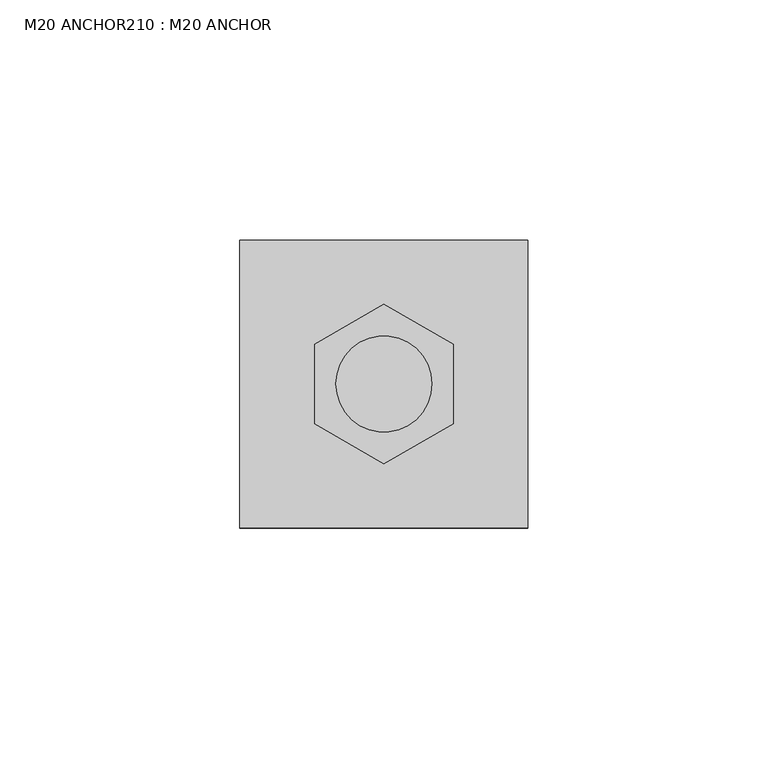
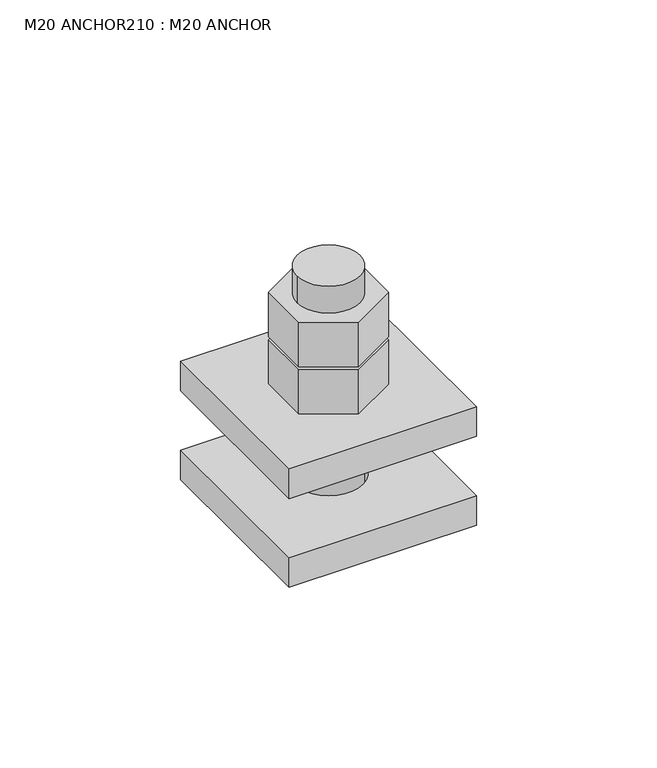
"""IFC4 building model written with IfcOpenShell, lengths in millimetres: fastener geometry, M20 ANCHOR210 : M20 ANCHOR."""

import ifcopenshell
import ifcopenshell.guid

model = None  # the IFC model being written
_history = None  # IfcOwnerHistory: only IFC2X3 demands one
_inside = {}  # id of a spatial element -> (the spatial element, [elements in it])
_under = {}  # id of a project, library or spatial element -> (it, [spatial elements below it])
_declared = {}  # id of a project -> (the project, [libraries it declares])
_typed = {}  # id of a type object -> (the type object, [elements of that type])
_made_of = {}  # id of a material, layer set ... -> (it, [elements and type objects made of it])


def new_model(schema):
    """Start an empty IFC model of exactly this schema.

    Asked for "IFC4X3", IfcOpenShell would pick the latest addendum, in which some entities
    have other attributes; the version numbers below select the first issue.
    IFC2X3 requires an IfcOwnerHistory on every rooted entity: one is made here for all.
    """
    global model, _history
    if schema == "IFC4X3":
        model = ifcopenshell.file(schema_version=(4, 3, 0, 0))
    else:
        model = ifcopenshell.file(schema=schema)
    _inside.clear()
    _under.clear()
    _declared.clear()
    _typed.clear()
    _made_of.clear()
    _history = None
    if model.schema == "IFC2X3":
        org = make("IfcOrganization", Name="unknown")
        user = make(
            "IfcPersonAndOrganization",
            ThePerson=make("IfcPerson", FamilyName="unknown"),
            TheOrganization=org,
        )
        app = make(
            "IfcApplication",
            ApplicationDeveloper=org,
            Version="unknown",
            ApplicationFullName="unknown",
            ApplicationIdentifier="unknown",
        )
        _history = make(
            "IfcOwnerHistory",
            OwningUser=user,
            OwningApplication=app,
            ChangeAction="ADDED",
            CreationDate=0,
        )
    return model


def make(cls, **values):
    """One entity of the class cls with the attributes given. An attribute that is None is left unset."""
    return model.create_entity(
        cls, **{name: value for name, value in values.items() if value is not None}
    )


def rooted(cls, **values):
    """An entity with a GlobalId (a new one), such as an element, a storey or a relation."""
    return make(cls, GlobalId=ifcopenshell.guid.new(), OwnerHistory=_history, **values)


def si_unit(unit_type, name, prefix=None):
    """IfcSIUnit, for example si_unit("LENGTHUNIT", "METRE", prefix="MILLI")."""
    return make("IfcSIUnit", UnitType=unit_type, Prefix=prefix, Name=name)


def assignment(units):
    """IfcUnitAssignment: the units of a project."""
    return None if units is None else make("IfcUnitAssignment", Units=units)


def point(xyz):
    """IfcCartesianPoint."""
    return None if xyz is None else make("IfcCartesianPoint", Coordinates=xyz)


def direction(xyz):
    """IfcDirection."""
    return None if xyz is None else make("IfcDirection", DirectionRatios=xyz)


def frame(location, z_axis=None, x_axis=None):
    """IfcAxis2Placement3D, a coordinate frame: its origin and axes. An axis left out is left unset."""
    return make(
        "IfcAxis2Placement3D",
        Location=point(location),
        Axis=direction(z_axis),
        RefDirection=direction(x_axis),
    )


def frame_2d(location, x_axis=None):
    """IfcAxis2Placement2D, a coordinate frame in the plane: its origin and x axis."""
    return make(
        "IfcAxis2Placement2D", Location=point(location), RefDirection=direction(x_axis)
    )


def origin():
    """The frame at (0, 0, 0) with its axes left unset."""
    return frame((0.0, 0.0, 0.0))


def place(relative_to, where):
    """IfcLocalPlacement: puts the frame where relative to a parent placement (None: the world)."""
    return make(
        "IfcLocalPlacement", PlacementRelTo=relative_to, RelativePlacement=where
    )


def context(
    kind, dimensions, precision=None, world=None, true_north=None, identifier=None
):
    """IfcGeometricRepresentationContext, for example the 3D "Model" context."""
    return make(
        "IfcGeometricRepresentationContext",
        ContextIdentifier=identifier,
        ContextType=kind,
        CoordinateSpaceDimension=dimensions,
        Precision=precision,
        WorldCoordinateSystem=world,
        TrueNorth=true_north,
    )


def project(units=None, contexts=None):
    """IfcProject with its units and contexts."""
    return rooted(
        "IfcProject",
        Name="project",
        RepresentationContexts=contexts,
        UnitsInContext=assignment(units),
    )


def spatial(cls, under=None, at=None, **own):
    """A site, building, storey or space (cls), placed at a placement, below another one or the project."""
    s = rooted(cls, ObjectPlacement=at, **own)
    if under is not None:
        _under.setdefault(under.id(), (under, []))[1].append(s)
    return s


def polyline(points):
    """IfcPolyline through the points."""
    return make("IfcPolyline", Points=[point(p) for p in points])


def circle_curve(where, radius):
    """IfcCircle in the frame where."""
    return make("IfcCircle", Position=where, Radius=radius)


def trimmed(basis, trim1, trim2, sense, master):
    """IfcTrimmedCurve: the piece of a basis curve between two trims."""
    return make(
        "IfcTrimmedCurve",
        BasisCurve=basis,
        Trim1=trim1,
        Trim2=trim2,
        SenseAgreement=sense,
        MasterRepresentation=master,
    )


def segment(curve, same_sense, transition):
    """IfcCompositeCurveSegment."""
    return make(
        "IfcCompositeCurveSegment",
        Transition=transition,
        SameSense=same_sense,
        ParentCurve=curve,
    )


def composite_curve(segments, self_intersect=None):
    """IfcCompositeCurve: segments joined end to end."""
    return make("IfcCompositeCurve", Segments=segments, SelfIntersect=self_intersect)


def outline(outer, holes=None, kind="AREA"):
    """IfcArbitraryClosedProfileDef: a profile drawn as a closed curve; with holes, ...WithVoids."""
    if holes is None:
        return make("IfcArbitraryClosedProfileDef", ProfileType=kind, OuterCurve=outer)
    return make(
        "IfcArbitraryProfileDefWithVoids",
        ProfileType=kind,
        OuterCurve=outer,
        InnerCurves=holes,
    )


def extrude(swept, where, along, depth):
    """IfcExtrudedAreaSolid: the profile swept, set in the frame where, extruded along a direction by depth."""
    return make(
        "IfcExtrudedAreaSolid",
        SweptArea=swept,
        Position=where,
        ExtrudedDirection=direction(along),
        Depth=depth,
    )


def shape(context_of_items, identifier, shape_type, items):
    """IfcShapeRepresentation: the items that make up one representation, for example the "Body"."""
    return make(
        "IfcShapeRepresentation",
        ContextOfItems=context_of_items,
        RepresentationIdentifier=identifier,
        RepresentationType=shape_type,
        Items=items,
    )


def source(mapping_origin, context_of_items, identifier, shape_type, items):
    """IfcRepresentationMap: a shape defined once, which mapped items show again and again."""
    return make(
        "IfcRepresentationMap",
        MappingOrigin=mapping_origin,
        MappedRepresentation=shape(context_of_items, identifier, shape_type, items),
    )


def transform(
    local_origin,
    x_axis=None,
    y_axis=None,
    z_axis=None,
    scale=None,
    scale2=None,
    scale3=None,
    uniform=True,
):
    """IfcCartesianTransformationOperator3D, or its non-uniform kind. x_axis, y_axis, z_axis: its Axis1, 2, 3."""
    if uniform:
        return make(
            "IfcCartesianTransformationOperator3D",
            Axis1=direction(x_axis),
            Axis2=direction(y_axis),
            LocalOrigin=point(local_origin),
            Scale=scale,
            Axis3=direction(z_axis),
        )
    return make(
        "IfcCartesianTransformationOperator3DnonUniform",
        Axis1=direction(x_axis),
        Axis2=direction(y_axis),
        LocalOrigin=point(local_origin),
        Scale=scale,
        Axis3=direction(z_axis),
        Scale2=scale2,
        Scale3=scale3,
    )


def mapped(mapping_source, mapping_target):
    """IfcMappedItem: shows the shape of a source again, moved by a transform."""
    return make(
        "IfcMappedItem", MappingSource=mapping_source, MappingTarget=mapping_target
    )


def made_of(thing, what):
    """Note that an element or type object is made of a material, layer set ...; save() writes the relation."""
    if what is not None:
        _made_of.setdefault(what.id(), (what, []))[1].append(thing)
    return thing


def element(
    cls,
    number,
    at=None,
    inside=None,
    cuts=None,
    type_object=None,
    material=None,
    context=None,
    identifier="Body",
    shape_type=None,
    held_by="IfcProductDefinitionShape",
    body=None,
    shapes=None,
    **own,
):
    """One element of the class cls, such as IfcWall. Its Tag is "e" and its number.

    at: its placement. inside: the storey or other place that contains it. cuts: it is an
    opening in that element (IfcRelVoidsElement). A single representation is given by context,
    identifier, shape_type and body (its items); several are given by shapes. held_by: the class
    of the entity that holds the representations. save() writes the other relations.
    """
    e = rooted(cls, Tag="e%d" % number, ObjectPlacement=at, **own)
    if body is not None:
        shapes = [shape(context, identifier, shape_type, body)]
    if shapes is not None:
        e.Representation = make(held_by, Representations=shapes)
    if inside is not None:
        _inside.setdefault(inside.id(), (inside, []))[1].append(e)
    if cuts is not None:
        rooted(
            "IfcRelVoidsElement", RelatingBuildingElement=cuts, RelatedOpeningElement=e
        )
    if type_object is not None:
        _typed.setdefault(type_object.id(), (type_object, []))[1].append(e)
    return made_of(e, material)


def aggregate(whole, parts):
    """IfcRelAggregates: a whole, such as a stair, and the parts it consists of."""
    return rooted("IfcRelAggregates", RelatingObject=whole, RelatedObjects=parts)


def save(model, path):
    """Write the relations noted so far, then the file.

    IfcRelAggregates (storeys below a building ...), IfcRelContainedInSpatialStructure (elements
    in a storey), IfcRelDefinesByType, IfcRelAssociatesMaterial and IfcRelDeclares: one each for
    every whole, place, type object, material and project.
    """
    for whole, parts in _under.values():
        aggregate(whole, parts)
    for where, things in _inside.values():
        rooted(
            "IfcRelContainedInSpatialStructure",
            RelatedElements=things,
            RelatingStructure=where,
        )
    for kind, things in _typed.values():
        rooted("IfcRelDefinesByType", RelatedObjects=things, RelatingType=kind)
    for what, things in _made_of.values():
        rooted("IfcRelAssociatesMaterial", RelatedObjects=things, RelatingMaterial=what)
    for by, libraries in _declared.values():
        rooted("IfcRelDeclares", RelatingContext=by, RelatedDefinitions=libraries)
    model.write(path)


def m20_anchor210_m20_anchor_1472a41f(model_context):
    return source(origin(), model_context, "Body", "SweptSolid", [
        extrude(outline(polyline([(8991.9144032, 22545.0952779), (8991.9144032, 22528.4582151), (8977.5062842, 22520.1396837), (8963.0981652, 22528.4582151), (8963.0981652, 22545.0952779), (8977.5062842, 22553.4138093), (8991.9144032, 22545.0952779)]), holes=[composite_curve([segment(trimmed(circle_curve(frame_2d((8977.5062842, 22536.7767465)), 10.0), [point((8967.5062842, 22536.7767465))], [point((8987.5062842, 22536.7767465))], True, "CARTESIAN"), True, "CONTINUOUS"), segment(trimmed(circle_curve(frame_2d((8977.5062842, 22536.7767465)), 10.0), [point((8987.5062842, 22536.7767465))], [point((8967.5062842, 22536.7767465))], True, "CARTESIAN"), True, "CONTINUOUS")], self_intersect=False)]), frame((0.0, 0.0, 246.0), z_axis=(0.0, 0.0, 1.0), x_axis=(1.0, 0.0, 0.0)), (0.0, 0.0, 1.0), 15.0),
        extrude(outline(polyline([(8991.9144032, 22545.0952779), (8991.9144032, 22528.4582151), (8977.5062842, 22520.1396837), (8963.0981652, 22528.4582151), (8963.0981652, 22545.0952779), (8977.5062842, 22553.4138093), (8991.9144032, 22545.0952779)]), holes=[composite_curve([segment(trimmed(circle_curve(frame_2d((8977.5062842, 22536.7767465)), 10.0), [point((8967.5062842, 22536.7767465))], [point((8987.5062842, 22536.7767465))], True, "CARTESIAN"), True, "CONTINUOUS"), segment(trimmed(circle_curve(frame_2d((8977.5062842, 22536.7767465)), 10.0), [point((8987.5062842, 22536.7767465))], [point((8967.5062842, 22536.7767465))], True, "CARTESIAN"), True, "CONTINUOUS")], self_intersect=False)]), frame((0.0, 0.0, 230.0), z_axis=(0.0, 0.0, 1.0), x_axis=(1.0, 0.0, 0.0)), (0.0, 0.0, 1.0), 15.0),
        extrude(outline(composite_curve([segment(trimmed(circle_curve(frame_2d((8977.5062842, 22536.7767465)), 10.0), [point((8967.5062842, 22536.7767465))], [point((8987.5062842, 22536.7767465))], False, "CARTESIAN"), True, "CONTINUOUS"), segment(trimmed(circle_curve(frame_2d((8977.5062842, 22536.7767465)), 10.0), [point((8987.5062842, 22536.7767465))], [point((8967.5062842, 22536.7767465))], False, "CARTESIAN"), True, "CONTINUOUS")], self_intersect=False)), frame((0.0, 0.0, 190.0), z_axis=(0.0, 0.0, 1.0), x_axis=(1.0, 0.0, 0.0)), (0.0, 0.0, 1.0), 80.0),
        extrude(outline(polyline([(9007.5062842, 22566.7767465), (9007.5062842, 22506.7767465), (8947.5062842, 22506.7767465), (8947.5062842, 22566.7767465), (9007.5062842, 22566.7767465)]), holes=[composite_curve([segment(trimmed(circle_curve(frame_2d((8977.5062842, 22536.7767465)), 11.0), [point((8966.5062842, 22536.7767465))], [point((8988.5062842, 22536.7767465))], True, "CARTESIAN"), True, "CONTINUOUS"), segment(trimmed(circle_curve(frame_2d((8977.5062842, 22536.7767465)), 11.0), [point((8988.5062842, 22536.7767465))], [point((8966.5062842, 22536.7767465))], True, "CARTESIAN"), True, "CONTINUOUS")], self_intersect=False)]), frame((0.0, 0.0, 190.0), z_axis=(0.0, 0.0, 1.0), x_axis=(1.0, 0.0, 0.0)), (0.0, 0.0, 1.0), 10.0),
        extrude(outline(polyline([(9007.5062842, 22566.7767465), (9007.5062842, 22506.7767465), (8947.5062842, 22506.7767465), (8947.5062842, 22566.7767465), (9007.5062842, 22566.7767465)]), holes=[composite_curve([segment(trimmed(circle_curve(frame_2d((8977.5062842, 22536.7767465)), 11.0), [point((8966.5062842, 22536.7767465))], [point((8988.5062842, 22536.7767465))], True, "CARTESIAN"), True, "CONTINUOUS"), segment(trimmed(circle_curve(frame_2d((8977.5062842, 22536.7767465)), 11.0), [point((8988.5062842, 22536.7767465))], [point((8966.5062842, 22536.7767465))], True, "CARTESIAN"), True, "CONTINUOUS")], self_intersect=False)]), frame((0.0, 0.0, 220.0), z_axis=(0.0, 0.0, 1.0), x_axis=(1.0, 0.0, 0.0)), (0.0, 0.0, 1.0), 10.0),
    ])


if __name__ == "__main__":
    model = new_model("IFC4")
    model_context = context("Model", 3, world=origin())
    ifc_project = project(units=[si_unit("LENGTHUNIT", "METRE", prefix="MILLI")], contexts=[model_context])
    site = spatial("IfcSite", under=ifc_project)
    building = spatial("IfcBuilding", under=site)
    placement = place(None, origin())
    m20_anchor210_m20_anchor_shape = m20_anchor210_m20_anchor_1472a41f(model_context)
    element("IfcFastener", 1, ObjectType="M20 ANCHOR210 : M20 ANCHOR", at=placement, inside=building, context=model_context, shape_type="MappedRepresentation", body=[
        mapped(m20_anchor210_m20_anchor_shape, transform((0.0, 0.0, 0.0), x_axis=(1.0, 0.0, 0.0), y_axis=(0.0, 1.0, 0.0), z_axis=(0.0, 0.0, 1.0))),
    ])
    save(model, "model.ifc")
